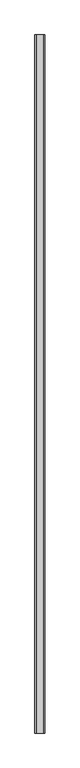
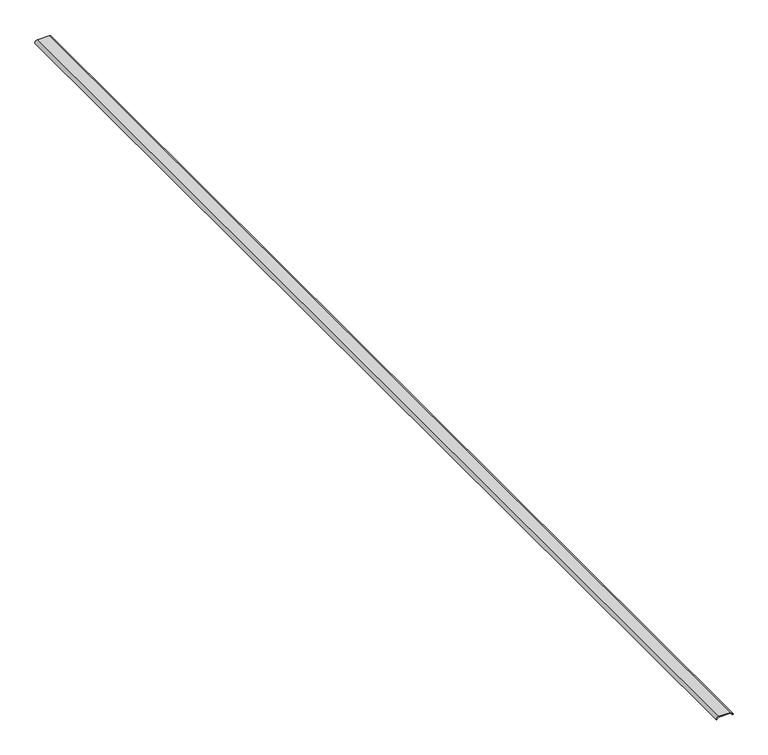
"""IFC4 building model written with IfcOpenShell, lengths in millimetres: proxy geometry, BEND PANEL3:BEND PANEL004:297576 : BEND PANEL3:BEND PANEL004:297576."""

from ifc_helpers import new_model, si_unit, point, frame, frame_2d, origin, place, context, project, spatial, polyline, circle_curve, trimmed, segment, composite_curve, outline, extrude, source, transform, mapped, element, save


def generic_models_48c50c2f(model_context):
    return source(origin(), model_context, "Body", "SweptSolid", [
        extrude(outline(composite_curve([segment(trimmed(circle_curve(frame_2d((42576.6119199, 10640.0084731)), 4.5989014), [point((42581.2108045, 10640.0209261))], [point((42576.6119199, 10635.4095717))], False, "CARTESIAN"), True, "CONTINUOUS"), segment(polyline([(42576.6119199, 10635.4095717), (42576.6119199, 10636.6001967)]), True, "CONTINUOUS"), segment(trimmed(circle_curve(frame_2d((42576.6119199, 10640.0084731)), 3.4082764), [point((42576.6119199, 10636.6001967))], [point((42580.0201795, 10640.0191867))], True, "CARTESIAN"), True, "CONTINUOUS"), segment(polyline([(42580.0201795, 10640.0191867), (42580.0201963, 10659.3736771)]), True, "CONTINUOUS"), segment(trimmed(circle_curve(frame_2d((42576.6119199, 10659.37368)), 3.4082764), [point((42580.0201963, 10659.3736771))], [point((42576.6119199, 10662.7819564))], True, "CARTESIAN"), True, "CONTINUOUS"), segment(polyline([(42576.6119199, 10662.7819564), (42576.6119199, 10663.9725814)]), True, "CONTINUOUS"), segment(trimmed(circle_curve(frame_2d((42576.6119199, 10659.37368)), 4.5989014), [point((42576.6119199, 10663.9725814))], [point((42581.2108213, 10659.373676))], False, "CARTESIAN"), True, "CONTINUOUS"), segment(polyline([(42581.2108213, 10659.373676), (42581.2108045, 10640.0209261)]), True, "CONTINUOUS")], self_intersect=False)), frame((0.0, -774.5581163, 0.0), z_axis=(0.0, 1.0, 0.0), x_axis=(0.0, 0.0, 1.0)), (0.0, 0.0, 1.0), 1999.85),
    ])


if __name__ == "__main__":
    model = new_model("IFC4")
    model_context = context("Model", 3, world=origin())
    ifc_project = project(units=[si_unit("LENGTHUNIT", "METRE", prefix="MILLI")], contexts=[model_context])
    site = spatial("IfcSite", under=ifc_project)
    building = spatial("IfcBuilding", under=site)
    placement = place(None, origin())
    generic_models_shape = generic_models_48c50c2f(model_context)
    element("IfcBuildingElementProxy", 1, Name="BEND PANEL3:BEND PANEL004:297576 : BEND PANEL3:BEND PANEL004:297576", ObjectType="BEND PANEL3:BEND PANEL004:297576 : BEND PANEL3:BEND PANEL004:297576", at=placement, inside=building, context=model_context, shape_type="MappedRepresentation", body=[
        mapped(generic_models_shape, transform((0.0, 0.0, 0.0), x_axis=(1.0, 0.0, 0.0), y_axis=(0.0, 1.0, 0.0), z_axis=(0.0, 0.0, 1.0))),
    ])
    save(model, "model.ifc")

# Revit data of these elements
# Type "BEND PANEL3:BEND PANEL004:297576 : BEND PANEL3:BEND PANEL004:297576"
#   NameOverride = "BEND PANEL3:BEND PANEL004:297576"
#   ObjectTypeOverride = "BEND PANEL3:BEND PANEL004"
#   Reference = "BEND PANEL004"
#   Category = "Generic Models"
#   Tag = "297576"
# Element 1 (IfcBuildingElementProxy, "BEND PANEL3:BEND PANEL004:297576 : BEND PANEL3:BEND PANEL004:297576")
#   Materials on its faces: "METAL PROFILE"
# Materials
#   "METAL PROFILE": class "Unassigned", colour RGB 128 128 128, transparency 0
